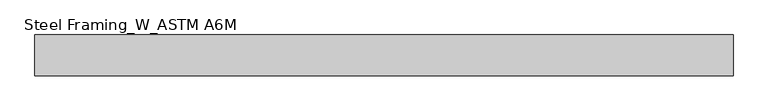
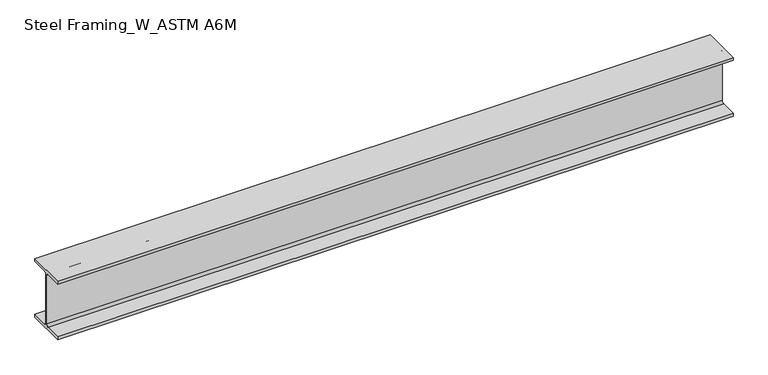
"""IFC4 building model written with IfcOpenShell, lengths in millimetres: beam geometry, Steel Framing_W_ASTM A6M : H_SB_AR_S02_W200x31.3_B6."""

from ifc_helpers import new_model, si_unit, point, frame, frame_2d, origin, place, context, project, spatial, polyline, circle_curve, trimmed, segment, composite_curve, outline, extrude, source, transform, mapped, element, save


def steel_framing_w_astm_a6m_6b735529(model_context):
    return source(origin(), model_context, "Body", "SweptSolid", [
        extrude(outline(composite_curve([segment(polyline([(67.0, -94.8), (67.0, -105.0), (-67.0, -105.0), (-67.0, -94.8), (-10.775, -94.8)]), True, "CONTINUOUS"), segment(trimmed(circle_curve(frame_2d((-10.775, -87.2)), 7.6), [point((-10.775, -94.8))], [point((-3.175, -87.2))], True, "CARTESIAN"), True, "CONTINUOUS"), segment(polyline([(-3.175, -87.2), (-3.175, 87.2)]), True, "CONTINUOUS"), segment(trimmed(circle_curve(frame_2d((-10.775, 87.2)), 7.6), [point((-3.175, 87.2))], [point((-10.775, 94.8))], True, "CARTESIAN"), True, "CONTINUOUS"), segment(polyline([(-10.775, 94.8), (-67.0, 94.8), (-67.0, 105.0), (67.0, 105.0), (67.0, 94.8), (10.775, 94.8)]), True, "CONTINUOUS"), segment(trimmed(circle_curve(frame_2d((10.775, 87.2)), 7.6), [point((10.775, 94.8))], [point((3.175, 87.2))], True, "CARTESIAN"), True, "CONTINUOUS"), segment(polyline([(3.175, 87.2), (3.175, -87.2)]), True, "CONTINUOUS"), segment(trimmed(circle_curve(frame_2d((10.775, -87.2)), 7.6), [point((3.175, -87.2))], [point((10.775, -94.8))], True, "CARTESIAN"), True, "CONTINUOUS"), segment(polyline([(10.775, -94.8), (67.0, -94.8)]), True, "CONTINUOUS")], self_intersect=False)), frame((-1140.8, 0.0, 0.0), z_axis=(1.0, 0.0, 0.0), x_axis=(0.0, 1.0, 0.0)), (0.0, 0.0, 1.0), 2292.6),
    ])


if __name__ == "__main__":
    model = new_model("IFC4")
    model_context = context("Model", 3, world=origin())
    ifc_project = project(units=[si_unit("LENGTHUNIT", "METRE", prefix="MILLI")], contexts=[model_context])
    site = spatial("IfcSite", under=ifc_project)
    building = spatial("IfcBuilding", under=site)
    placement = place(None, origin())
    steel_framing_w_astm_a6m_shape = steel_framing_w_astm_a6m_6b735529(model_context)
    element("IfcBeam", 1, ObjectType="Steel Framing_W_ASTM A6M : H_SB_AR_S02_W200x31.3_B6", at=placement, inside=building, context=model_context, shape_type="MappedRepresentation", body=[
        mapped(steel_framing_w_astm_a6m_shape, transform((0.0, 0.0, 0.0), x_axis=(1.0, 0.0, 0.0), y_axis=(0.0, 1.0, 0.0), z_axis=(0.0, 0.0, 1.0))),
    ])
    save(model, "model.ifc")

# Revit data of these elements
# Type "Steel Framing_W_ASTM A6M : H_SB_AR_S02_W200x31.3_B6"
#   Type Mark = "B6"
#   Section Name Key = "W8x21"
#   Width = 13.4 cm
#   Web Thickness = 0.635 cm
#   Web Fillet = 0.76 cm
#   Warping Constant = 40800.0 cm⁶
#   Torsional Moment of Inertia = 11.70 cm⁴
#   Section Area = 39.7 cm²
#   Plastic Modulus weak axis = 93.2 cm³
#   Plastic Modulus strong axis = 334.0 cm³
#   Perimeter = 0.93 m²/m
#   Nominal Weight = 31.30 kgf/m
#   Moment of Inertia weak axis = 407.00 cm⁴
#   Moment of Inertia strong axis = 3130.00 cm⁴
#   Height = 21.0 cm
#   Flange Thickness = 1.02 cm
#   Elastic Modulus weak axis = 60.8 cm³
#   Elastic Modulus strong axis = 298.0 cm³
#   Centroid Vertical = 10.5 cm
#   Centroid Horizontal = 6.7 cm
#   Length [instance default] = 1500 mm
#   Structural Material [instance default] = Steel, 45-345
#   Bolt Spacing = 0
#   Assembly Code = ""
# Element 1 (IfcBeam, "Steel Framing_W_ASTM A6M : H_SB_AR_S02_W200x31.3_B6")
#   Materials on its faces: "Steel, 45-345"
# Materials
#   "Steel, 45-345": class "Metal", colour RGB 189 187 185, transparency 0, Description = "Steel 345 MPa", Cost = 0
